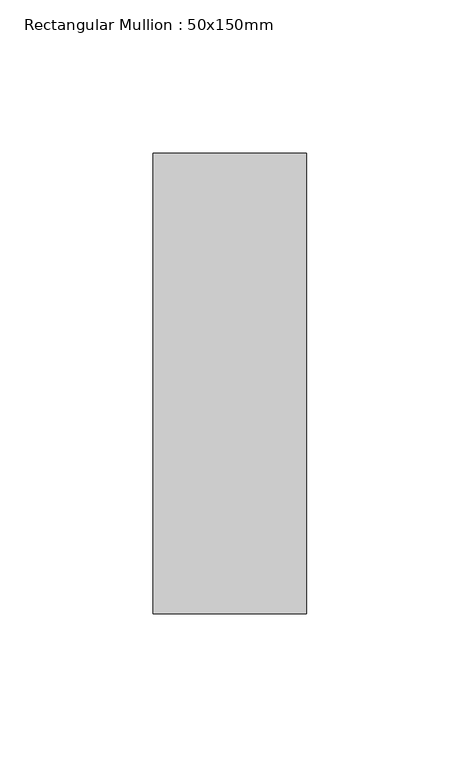
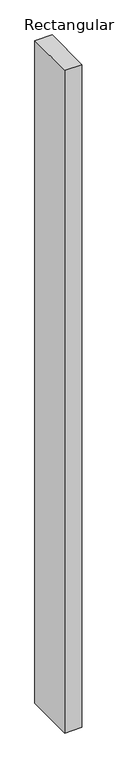
"""IFC4 building model written with IfcOpenShell, lengths in millimetres: member geometry, Rectangular Mullion : 50x150mm."""

from ifc_helpers import new_model, si_unit, frame, origin, place, context, project, spatial, polyline, outline, extrude, source, transform, mapped, element, save


def rectangular_mullion_50x150mm_81e5845b(model_context):
    return source(origin(), model_context, "Body", "SweptSolid", [
        extrude(outline(polyline([(25.0, 75.0), (25.0, -75.0), (-25.0, -75.0), (-25.0, 75.0), (25.0, 75.0)])), frame((0.0, 0.0, -2034.1016494), z_axis=(0.0, 0.0, 1.0), x_axis=(1.0, 0.0, 0.0)), (0.0, 0.0, 1.0), 2034.1016494),
    ])


if __name__ == "__main__":
    model = new_model("IFC4")
    model_context = context("Model", 3, world=origin())
    ifc_project = project(units=[si_unit("LENGTHUNIT", "METRE", prefix="MILLI")], contexts=[model_context])
    site = spatial("IfcSite", under=ifc_project)
    building = spatial("IfcBuilding", under=site)
    placement = place(None, origin())
    rectangular_mullion_50x150mm_shape = rectangular_mullion_50x150mm_81e5845b(model_context)
    element("IfcMember", 1, ObjectType="Rectangular Mullion : 50x150mm", at=placement, inside=building, context=model_context, shape_type="MappedRepresentation", body=[
        mapped(rectangular_mullion_50x150mm_shape, transform((0.0, 0.0, 0.0), x_axis=(1.0, 0.0, 0.0), y_axis=(0.0, 1.0, 0.0), z_axis=(0.0, 0.0, 1.0))),
    ])
    save(model, "model.ifc")

# Revit data of these elements
# Type "Rectangular Mullion : 50x150mm"
#   Keynote = "H11"
#   built-in parameter 1007304 = 0.492126 (stored number, unit not read)
#   built-in parameter 1007301 = 0.082021 (stored number, unit not read)
#   built-in parameter 1007300 = 0.082021 (stored number, unit not read)
# Element 1 (IfcMember, "Rectangular Mullion : 50x150mm")
#   Materials on its faces: "Aluminium"
# Materials
#   "Aluminium": class "Metal", colour RGB 247 247 247, transparency 0, Description = "Aluminium 6061", Cost = 0
